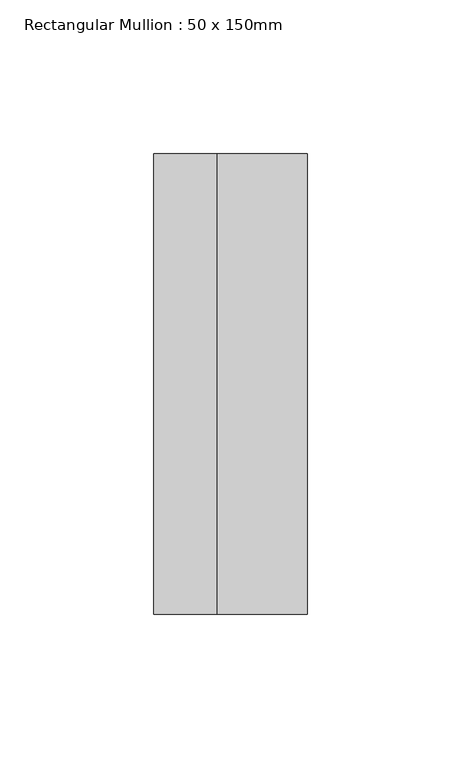
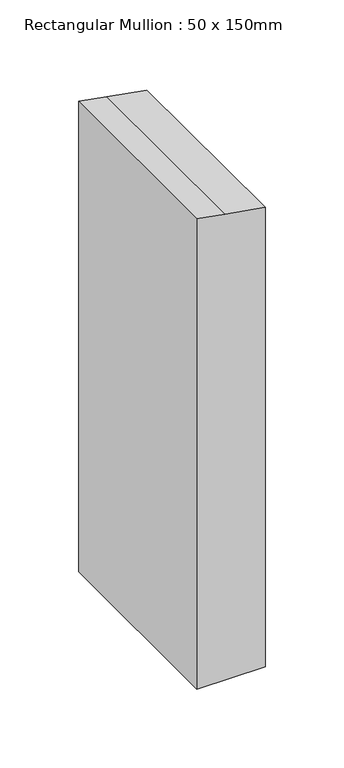
"""IFC4 building model written with IfcOpenShell, lengths in millimetres: member geometry, Rectangular Mullion : 50 x 150mm."""

from ifc_helpers import new_model, si_unit, frame, origin, place, context, project, spatial, polyline, outline, extrude, source, transform, mapped, element, save


def rectangular_mullion_50_x_150mm_bc448f9a(model_context):
    return source(origin(), model_context, "Body", "SweptSolid", [
        extrude(outline(polyline([(-4.7938398, 25.0), (0.3798062, -4.3412044), (4.0225092, -25.0), (-360.7536619, -25.0), (-360.7536619, 25.0), (-4.7938398, 25.0)])), frame((0.0, -75.0, 0.0), z_axis=(0.0, 1.0, 0.0), x_axis=(0.0, 0.0, 1.0)), (0.0, 0.0, 1.0), 150.0),
    ])


if __name__ == "__main__":
    model = new_model("IFC4")
    model_context = context("Model", 3, world=origin())
    ifc_project = project(units=[si_unit("LENGTHUNIT", "METRE", prefix="MILLI")], contexts=[model_context])
    site = spatial("IfcSite", under=ifc_project)
    building = spatial("IfcBuilding", under=site)
    placement = place(None, origin())
    rectangular_mullion_50_x_150mm_shape = rectangular_mullion_50_x_150mm_bc448f9a(model_context)
    element("IfcMember", 1, ObjectType="Rectangular Mullion : 50 x 150mm", at=placement, inside=building, context=model_context, shape_type="MappedRepresentation", body=[
        mapped(rectangular_mullion_50_x_150mm_shape, transform((0.0, 0.0, 0.0), x_axis=(1.0, 0.0, 0.0), y_axis=(0.0, 1.0, 0.0), z_axis=(0.0, 0.0, 1.0))),
    ])
    save(model, "model.ifc")

# Revit data of these elements
# Type "Rectangular Mullion : 50 x 150mm"
#   built-in parameter 1007304 = 0.492126 (stored number, unit not read)
#   built-in parameter 1007301 = 0.082021 (stored number, unit not read)
#   built-in parameter 1007300 = 0.082021 (stored number, unit not read)
# Element 1 (IfcMember, "Rectangular Mullion : 50 x 150mm")
#   Materials on its faces: "Aluminium"
# Materials
#   "Aluminium": class "Metal", colour RGB 247 247 247, transparency 0, Description = "Aluminium 6061", Cost = 0
